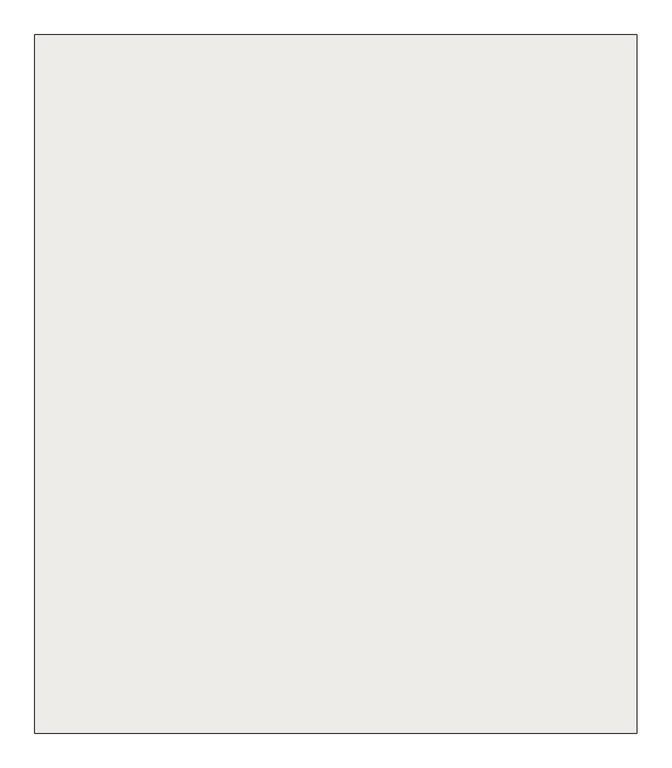
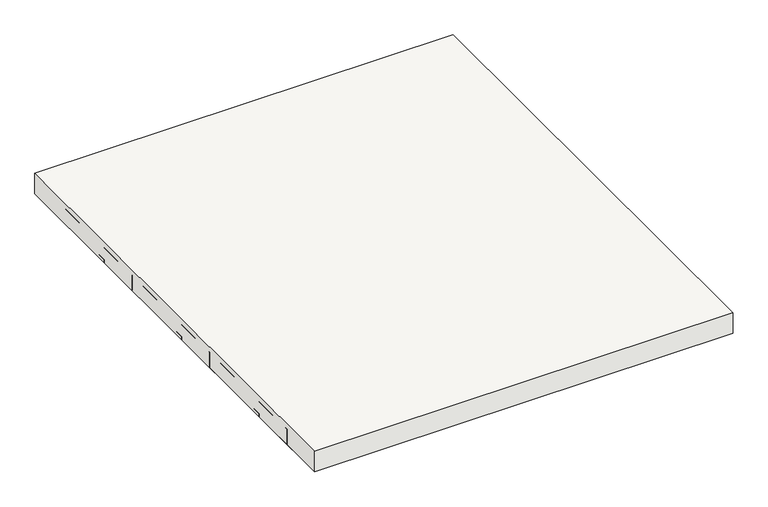
"""IFC4 building model written with IfcOpenShell, lengths in millimetres: slab geometry, Pano 3 (16 cm)."""

from ifc_helpers import new_model, si_unit, origin, origin_with_axes, place, context, project, spatial, polyline, outline, extrude, source, transform, mapped, element, save


def slab_b37928b6(model_context):
    return source(origin(), model_context, "Body", "SweptSolid", [
        extrude(outline(polyline([(-860.0, 9100.0), (2255.00107, 9100.0), (2255.00107, 5490.0), (-860.0, 5490.0), (-860.0, 9100.0)])), origin_with_axes(), (0.0, 0.0, 1.0), 160.0),
        extrude(outline(polyline([(-860.0, 5704.0), (-860.0, 5844.0), (2255.00107, 5844.0), (2255.00107, 5704.0), (-860.0, 5704.0)])), origin_with_axes(), (0.0, 0.0, 1.0), 24.0),
        extrude(outline(polyline([(-860.0, 6844.0), (-860.0, 7204.0), (-365.0, 7204.0), (-365.0, 6844.0), (-860.0, 6844.0)])), origin_with_axes(), (0.0, 0.0, 1.0), 120.0),
        extrude(outline(polyline([(640.0, 6344.0), (640.0, 6704.0), (1135.0, 6704.0), (1135.0, 6344.0), (640.0, 6344.0)])), origin_with_axes(), (0.0, 0.0, 1.0), 120.0),
        extrude(outline(polyline([(-360.0, 5844.0), (-360.0, 6204.0), (135.0, 6204.0), (135.0, 5844.0), (-360.0, 5844.0)])), origin_with_axes(), (0.0, 0.0, 1.0), 120.0),
        extrude(outline(polyline([(1640.0, 7844.0), (1640.0, 8204.0), (2135.0, 8204.0), (2135.0, 7844.0), (1640.0, 7844.0)])), origin_with_axes(), (0.0, 0.0, 1.0), 120.0),
        extrude(outline(polyline([(640.0, 6844.0), (640.0, 7204.0), (1135.0, 7204.0), (1135.0, 6844.0), (640.0, 6844.0)])), origin_with_axes(), (0.0, 0.0, 1.0), 120.0),
        extrude(outline(polyline([(-860.0, 7704.0), (-860.0, 7844.0), (2255.00107, 7844.0), (2255.00107, 7704.0), (-860.0, 7704.0)])), origin_with_axes(), (0.0, 0.0, 1.0), 24.0),
        extrude(outline(polyline([(1140.0, 6844.0), (1140.0, 7204.0), (1635.0, 7204.0), (1635.0, 6844.0), (1140.0, 6844.0)])), origin_with_axes(), (0.0, 0.0, 1.0), 120.0),
        extrude(outline(polyline([(140.0, 6344.0), (140.0, 6704.0), (635.0, 6704.0), (635.0, 6344.0), (140.0, 6344.0)])), origin_with_axes(), (0.0, 0.0, 1.0), 120.0),
        extrude(outline(polyline([(1140.0, 7844.0), (1140.0, 8204.0), (1635.0, 8204.0), (1635.0, 7844.0), (1140.0, 7844.0)])), origin_with_axes(), (0.0, 0.0, 1.0), 120.0),
        extrude(outline(polyline([(2140.0, 8344.0), (2140.0, 8704.0), (2250.00107, 8704.0), (2250.00107, 8344.0), (2140.0, 8344.0)])), origin_with_axes(), (0.0, 0.0, 1.0), 120.0),
        extrude(outline(polyline([(2140.0, 7844.0), (2140.0, 8204.0), (2250.00107, 8204.0), (2250.00107, 7844.0), (2140.0, 7844.0)])), origin_with_axes(), (0.0, 0.0, 1.0), 120.0),
        extrude(outline(polyline([(1640.0, 6844.0), (1640.0, 7204.0), (2135.0, 7204.0), (2135.0, 6844.0), (1640.0, 6844.0)])), origin_with_axes(), (0.0, 0.0, 1.0), 120.0),
        extrude(outline(polyline([(-860.0, 7344.0), (-860.0, 7704.0), (-365.0, 7704.0), (-365.0, 7344.0), (-860.0, 7344.0)])), origin_with_axes(), (0.0, 0.0, 1.0), 120.0),
        extrude(outline(polyline([(140.0, 8344.0), (140.0, 8704.0), (635.0, 8704.0), (635.0, 8344.0), (140.0, 8344.0)])), origin_with_axes(), (0.0, 0.0, 1.0), 120.0),
        extrude(outline(polyline([(-860.0, 6704.0), (-860.0, 6844.0), (2255.00107, 6844.0), (2255.00107, 6704.0), (-860.0, 6704.0)])), origin_with_axes(), (0.0, 0.0, 1.0), 24.0),
        extrude(outline(polyline([(1640.0, 5844.0), (1640.0, 6204.0), (2135.0, 6204.0), (2135.0, 5844.0), (1640.0, 5844.0)])), origin_with_axes(), (0.0, 0.0, 1.0), 120.0),
        extrude(outline(polyline([(640.0, 5844.0), (640.0, 6204.0), (1135.0, 6204.0), (1135.0, 5844.0), (640.0, 5844.0)])), origin_with_axes(), (0.0, 0.0, 1.0), 120.0),
        extrude(outline(polyline([(-360.0, 6844.0), (-360.0, 7204.0), (135.0, 7204.0), (135.0, 6844.0), (-360.0, 6844.0)])), origin_with_axes(), (0.0, 0.0, 1.0), 120.0),
        extrude(outline(polyline([(-860.0, 8704.0), (-860.0, 8844.0), (2255.00107, 8844.0), (2255.00107, 8704.0), (-860.0, 8704.0)])), origin_with_axes(), (0.0, 0.0, 1.0), 24.0),
        extrude(outline(polyline([(1640.0, 8344.0), (1640.0, 8704.0), (2135.0, 8704.0), (2135.0, 8344.0), (1640.0, 8344.0)])), origin_with_axes(), (0.0, 0.0, 1.0), 120.0),
        extrude(outline(polyline([(-860.0, 8344.0), (-860.0, 8704.0), (-365.0, 8704.0), (-365.0, 8344.0), (-860.0, 8344.0)])), origin_with_axes(), (0.0, 0.0, 1.0), 120.0),
        extrude(outline(polyline([(140.0, 6844.0), (140.0, 7204.0), (635.0, 7204.0), (635.0, 6844.0), (140.0, 6844.0)])), origin_with_axes(), (0.0, 0.0, 1.0), 120.0),
        extrude(outline(polyline([(140.0, 7344.0), (140.0, 7704.0), (635.0, 7704.0), (635.0, 7344.0), (140.0, 7344.0)])), origin_with_axes(), (0.0, 0.0, 1.0), 120.0),
        extrude(outline(polyline([(-360.0, 7344.0), (-360.0, 7704.0), (135.0, 7704.0), (135.0, 7344.0), (-360.0, 7344.0)])), origin_with_axes(), (0.0, 0.0, 1.0), 120.0),
        extrude(outline(polyline([(1140.0, 5844.0), (1140.0, 6204.0), (1635.0, 6204.0), (1635.0, 5844.0), (1140.0, 5844.0)])), origin_with_axes(), (0.0, 0.0, 1.0), 120.0),
        extrude(outline(polyline([(2140.0, 7344.0), (2140.0, 7704.0), (2250.00107, 7704.0), (2250.00107, 7344.0), (2140.0, 7344.0)])), origin_with_axes(), (0.0, 0.0, 1.0), 120.0),
        extrude(outline(polyline([(-860.0, 6344.0), (-860.0, 6704.0), (-365.0, 6704.0), (-365.0, 6344.0), (-860.0, 6344.0)])), origin_with_axes(), (0.0, 0.0, 1.0), 120.0),
        extrude(outline(polyline([(2140.0, 5844.0), (2140.0, 6204.0), (2250.00107, 6204.0), (2250.00107, 5844.0), (2140.0, 5844.0)])), origin_with_axes(), (0.0, 0.0, 1.0), 120.0),
        extrude(outline(polyline([(140.0, 5844.0), (140.0, 6204.0), (635.0, 6204.0), (635.0, 5844.0), (140.0, 5844.0)])), origin_with_axes(), (0.0, 0.0, 1.0), 120.0),
        extrude(outline(polyline([(640.0, 7344.0), (640.0, 7704.0), (1135.0, 7704.0), (1135.0, 7344.0), (640.0, 7344.0)])), origin_with_axes(), (0.0, 0.0, 1.0), 120.0),
        extrude(outline(polyline([(-860.0, 5844.0), (-860.0, 6204.0), (-365.0, 6204.0), (-365.0, 5844.0), (-860.0, 5844.0)])), origin_with_axes(), (0.0, 0.0, 1.0), 120.0),
        extrude(outline(polyline([(-860.0, 7204.0), (-860.0, 7344.0), (2255.00107, 7344.0), (2255.00107, 7204.0), (-860.0, 7204.0)])), origin_with_axes(), (0.0, 0.0, 1.0), 24.0),
        extrude(outline(polyline([(2140.0, 6344.0), (2140.0, 6704.0), (2250.00107, 6704.0), (2250.00107, 6344.0), (2140.0, 6344.0)])), origin_with_axes(), (0.0, 0.0, 1.0), 120.0),
        extrude(outline(polyline([(-860.0, 8204.0), (-860.0, 8344.0), (2255.00107, 8344.0), (2255.00107, 8204.0), (-860.0, 8204.0)])), origin_with_axes(), (0.0, 0.0, 1.0), 24.0),
        extrude(outline(polyline([(-860.0, 7844.0), (-860.0, 8204.0), (-365.0, 8204.0), (-365.0, 7844.0), (-860.0, 7844.0)])), origin_with_axes(), (0.0, 0.0, 1.0), 120.0),
        extrude(outline(polyline([(1140.0, 7344.0), (1140.0, 7704.0), (1635.0, 7704.0), (1635.0, 7344.0), (1140.0, 7344.0)])), origin_with_axes(), (0.0, 0.0, 1.0), 120.0),
        extrude(outline(polyline([(140.0, 7844.0), (140.0, 8204.0), (635.0, 8204.0), (635.0, 7844.0), (140.0, 7844.0)])), origin_with_axes(), (0.0, 0.0, 1.0), 120.0),
        extrude(outline(polyline([(640.0, 7844.0), (640.0, 8204.0), (1135.0, 8204.0), (1135.0, 7844.0), (640.0, 7844.0)])), origin_with_axes(), (0.0, 0.0, 1.0), 120.0),
        extrude(outline(polyline([(1140.0, 8344.0), (1140.0, 8704.0), (1635.0, 8704.0), (1635.0, 8344.0), (1140.0, 8344.0)])), origin_with_axes(), (0.0, 0.0, 1.0), 120.0),
        extrude(outline(polyline([(-360.0, 6344.0), (-360.0, 6704.0), (135.0, 6704.0), (135.0, 6344.0), (-360.0, 6344.0)])), origin_with_axes(), (0.0, 0.0, 1.0), 120.0),
        extrude(outline(polyline([(640.0, 8344.0), (640.0, 8704.0), (1135.0, 8704.0), (1135.0, 8344.0), (640.0, 8344.0)])), origin_with_axes(), (0.0, 0.0, 1.0), 120.0),
        extrude(outline(polyline([(1640.0, 6344.0), (1640.0, 6704.0), (2135.0, 6704.0), (2135.0, 6344.0), (1640.0, 6344.0)])), origin_with_axes(), (0.0, 0.0, 1.0), 120.0),
        extrude(outline(polyline([(2140.0, 6844.0), (2140.0, 7204.0), (2250.00107, 7204.0), (2250.00107, 6844.0), (2140.0, 6844.0)])), origin_with_axes(), (0.0, 0.0, 1.0), 120.0),
        extrude(outline(polyline([(1140.0, 6344.0), (1140.0, 6704.0), (1635.0, 6704.0), (1635.0, 6344.0), (1140.0, 6344.0)])), origin_with_axes(), (0.0, 0.0, 1.0), 120.0),
        extrude(outline(polyline([(-360.0, 8344.0), (-360.0, 8704.0), (135.0, 8704.0), (135.0, 8344.0), (-360.0, 8344.0)])), origin_with_axes(), (0.0, 0.0, 1.0), 120.0),
        extrude(outline(polyline([(-860.0, 6204.0), (-860.0, 6344.0), (2255.00107, 6344.0), (2255.00107, 6204.0), (-860.0, 6204.0)])), origin_with_axes(), (0.0, 0.0, 1.0), 24.0),
        extrude(outline(polyline([(1640.0, 7344.0), (1640.0, 7704.0), (2135.0, 7704.0), (2135.0, 7344.0), (1640.0, 7344.0)])), origin_with_axes(), (0.0, 0.0, 1.0), 120.0),
        extrude(outline(polyline([(-360.0, 7844.0), (-360.0, 8204.0), (135.0, 8204.0), (135.0, 7844.0), (-360.0, 7844.0)])), origin_with_axes(), (0.0, 0.0, 1.0), 120.0),
    ])


if __name__ == "__main__":
    model = new_model("IFC4")
    model_context = context("Model", 3, world=origin())
    ifc_project = project(units=[si_unit("LENGTHUNIT", "METRE", prefix="MILLI")], contexts=[model_context])
    site = spatial("IfcSite", under=ifc_project)
    building = spatial("IfcBuilding", under=site)
    placement = place(None, origin())
    slab_shape = slab_b37928b6(model_context)
    element("IfcSlab", 1, ObjectType="Pano 3 (16 cm)", at=placement, inside=building, context=model_context, shape_type="MappedRepresentation", body=[
        mapped(slab_shape, transform((0.0, 0.0, 0.0), x_axis=(1.0, 0.0, 0.0), y_axis=(0.0, 1.0, 0.0), z_axis=(0.0, 0.0, 1.0))),
    ])
    save(model, "model.ifc")

# Revit data of these elements
# Element 1 (IfcSlab, "Pano 3 (16 cm)")
#   Materials on its faces: "Molde de poliestireno", "Concreto armado", "RGB 168-169-158"
# Materials
#   "Molde de poliestireno": class "Não atribuído", colour RGB 255 255 255, transparency 0
#   "Concreto armado": class "Não atribuído", colour RGB 168 169 158, transparency 0
#   "RGB 168-169-158": class "Não atribuído", colour RGB 168 169 158, transparency 0
